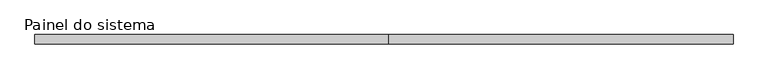
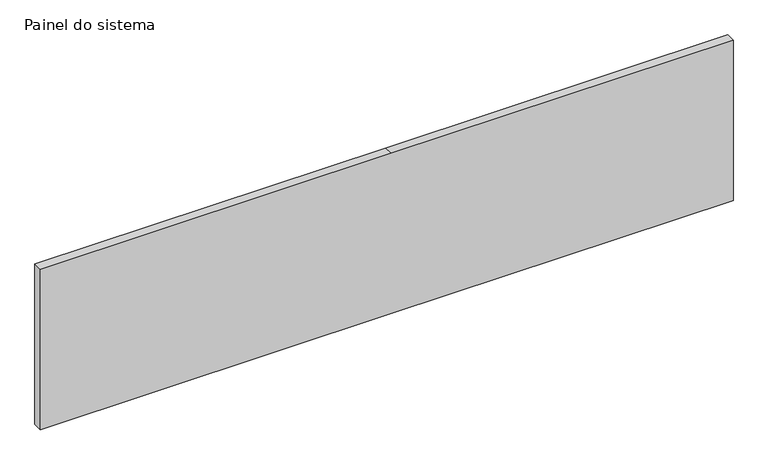
"""IFC4 building model written with IfcOpenShell, lengths in millimetres: plate geometry, Painel do sistema : Envidraçado."""

import ifcopenshell
import ifcopenshell.guid

model = None  # the IFC model being written
_history = None  # IfcOwnerHistory: only IFC2X3 demands one
_inside = {}  # id of a spatial element -> (the spatial element, [elements in it])
_under = {}  # id of a project, library or spatial element -> (it, [spatial elements below it])
_declared = {}  # id of a project -> (the project, [libraries it declares])
_typed = {}  # id of a type object -> (the type object, [elements of that type])
_made_of = {}  # id of a material, layer set ... -> (it, [elements and type objects made of it])


def new_model(schema):
    """Start an empty IFC model of exactly this schema.

    Asked for "IFC4X3", IfcOpenShell would pick the latest addendum, in which some entities
    have other attributes; the version numbers below select the first issue.
    IFC2X3 requires an IfcOwnerHistory on every rooted entity: one is made here for all.
    """
    global model, _history
    if schema == "IFC4X3":
        model = ifcopenshell.file(schema_version=(4, 3, 0, 0))
    else:
        model = ifcopenshell.file(schema=schema)
    _inside.clear()
    _under.clear()
    _declared.clear()
    _typed.clear()
    _made_of.clear()
    _history = None
    if model.schema == "IFC2X3":
        org = make("IfcOrganization", Name="unknown")
        user = make(
            "IfcPersonAndOrganization",
            ThePerson=make("IfcPerson", FamilyName="unknown"),
            TheOrganization=org,
        )
        app = make(
            "IfcApplication",
            ApplicationDeveloper=org,
            Version="unknown",
            ApplicationFullName="unknown",
            ApplicationIdentifier="unknown",
        )
        _history = make(
            "IfcOwnerHistory",
            OwningUser=user,
            OwningApplication=app,
            ChangeAction="ADDED",
            CreationDate=0,
        )
    return model


def make(cls, **values):
    """One entity of the class cls with the attributes given. An attribute that is None is left unset."""
    return model.create_entity(
        cls, **{name: value for name, value in values.items() if value is not None}
    )


def rooted(cls, **values):
    """An entity with a GlobalId (a new one), such as an element, a storey or a relation."""
    return make(cls, GlobalId=ifcopenshell.guid.new(), OwnerHistory=_history, **values)


def si_unit(unit_type, name, prefix=None):
    """IfcSIUnit, for example si_unit("LENGTHUNIT", "METRE", prefix="MILLI")."""
    return make("IfcSIUnit", UnitType=unit_type, Prefix=prefix, Name=name)


def assignment(units):
    """IfcUnitAssignment: the units of a project."""
    return None if units is None else make("IfcUnitAssignment", Units=units)


def point(xyz):
    """IfcCartesianPoint."""
    return None if xyz is None else make("IfcCartesianPoint", Coordinates=xyz)


def direction(xyz):
    """IfcDirection."""
    return None if xyz is None else make("IfcDirection", DirectionRatios=xyz)


def frame(location, z_axis=None, x_axis=None):
    """IfcAxis2Placement3D, a coordinate frame: its origin and axes. An axis left out is left unset."""
    return make(
        "IfcAxis2Placement3D",
        Location=point(location),
        Axis=direction(z_axis),
        RefDirection=direction(x_axis),
    )


def origin():
    """The frame at (0, 0, 0) with its axes left unset."""
    return frame((0.0, 0.0, 0.0))


def place(relative_to, where):
    """IfcLocalPlacement: puts the frame where relative to a parent placement (None: the world)."""
    return make(
        "IfcLocalPlacement", PlacementRelTo=relative_to, RelativePlacement=where
    )


def context(
    kind, dimensions, precision=None, world=None, true_north=None, identifier=None
):
    """IfcGeometricRepresentationContext, for example the 3D "Model" context."""
    return make(
        "IfcGeometricRepresentationContext",
        ContextIdentifier=identifier,
        ContextType=kind,
        CoordinateSpaceDimension=dimensions,
        Precision=precision,
        WorldCoordinateSystem=world,
        TrueNorth=true_north,
    )


def project(units=None, contexts=None):
    """IfcProject with its units and contexts."""
    return rooted(
        "IfcProject",
        Name="project",
        RepresentationContexts=contexts,
        UnitsInContext=assignment(units),
    )


def spatial(cls, under=None, at=None, **own):
    """A site, building, storey or space (cls), placed at a placement, below another one or the project."""
    s = rooted(cls, ObjectPlacement=at, **own)
    if under is not None:
        _under.setdefault(under.id(), (under, []))[1].append(s)
    return s


def polyline(points):
    """IfcPolyline through the points."""
    return make("IfcPolyline", Points=[point(p) for p in points])


def outline(outer, holes=None, kind="AREA"):
    """IfcArbitraryClosedProfileDef: a profile drawn as a closed curve; with holes, ...WithVoids."""
    if holes is None:
        return make("IfcArbitraryClosedProfileDef", ProfileType=kind, OuterCurve=outer)
    return make(
        "IfcArbitraryProfileDefWithVoids",
        ProfileType=kind,
        OuterCurve=outer,
        InnerCurves=holes,
    )


def extrude(swept, where, along, depth):
    """IfcExtrudedAreaSolid: the profile swept, set in the frame where, extruded along a direction by depth."""
    return make(
        "IfcExtrudedAreaSolid",
        SweptArea=swept,
        Position=where,
        ExtrudedDirection=direction(along),
        Depth=depth,
    )


def shape(context_of_items, identifier, shape_type, items):
    """IfcShapeRepresentation: the items that make up one representation, for example the "Body"."""
    return make(
        "IfcShapeRepresentation",
        ContextOfItems=context_of_items,
        RepresentationIdentifier=identifier,
        RepresentationType=shape_type,
        Items=items,
    )


def source(mapping_origin, context_of_items, identifier, shape_type, items):
    """IfcRepresentationMap: a shape defined once, which mapped items show again and again."""
    return make(
        "IfcRepresentationMap",
        MappingOrigin=mapping_origin,
        MappedRepresentation=shape(context_of_items, identifier, shape_type, items),
    )


def transform(
    local_origin,
    x_axis=None,
    y_axis=None,
    z_axis=None,
    scale=None,
    scale2=None,
    scale3=None,
    uniform=True,
):
    """IfcCartesianTransformationOperator3D, or its non-uniform kind. x_axis, y_axis, z_axis: its Axis1, 2, 3."""
    if uniform:
        return make(
            "IfcCartesianTransformationOperator3D",
            Axis1=direction(x_axis),
            Axis2=direction(y_axis),
            LocalOrigin=point(local_origin),
            Scale=scale,
            Axis3=direction(z_axis),
        )
    return make(
        "IfcCartesianTransformationOperator3DnonUniform",
        Axis1=direction(x_axis),
        Axis2=direction(y_axis),
        LocalOrigin=point(local_origin),
        Scale=scale,
        Axis3=direction(z_axis),
        Scale2=scale2,
        Scale3=scale3,
    )


def mapped(mapping_source, mapping_target):
    """IfcMappedItem: shows the shape of a source again, moved by a transform."""
    return make(
        "IfcMappedItem", MappingSource=mapping_source, MappingTarget=mapping_target
    )


def made_of(thing, what):
    """Note that an element or type object is made of a material, layer set ...; save() writes the relation."""
    if what is not None:
        _made_of.setdefault(what.id(), (what, []))[1].append(thing)
    return thing


def element(
    cls,
    number,
    at=None,
    inside=None,
    cuts=None,
    type_object=None,
    material=None,
    context=None,
    identifier="Body",
    shape_type=None,
    held_by="IfcProductDefinitionShape",
    body=None,
    shapes=None,
    **own,
):
    """One element of the class cls, such as IfcWall. Its Tag is "e" and its number.

    at: its placement. inside: the storey or other place that contains it. cuts: it is an
    opening in that element (IfcRelVoidsElement). A single representation is given by context,
    identifier, shape_type and body (its items); several are given by shapes. held_by: the class
    of the entity that holds the representations. save() writes the other relations.
    """
    e = rooted(cls, Tag="e%d" % number, ObjectPlacement=at, **own)
    if body is not None:
        shapes = [shape(context, identifier, shape_type, body)]
    if shapes is not None:
        e.Representation = make(held_by, Representations=shapes)
    if inside is not None:
        _inside.setdefault(inside.id(), (inside, []))[1].append(e)
    if cuts is not None:
        rooted(
            "IfcRelVoidsElement", RelatingBuildingElement=cuts, RelatedOpeningElement=e
        )
    if type_object is not None:
        _typed.setdefault(type_object.id(), (type_object, []))[1].append(e)
    return made_of(e, material)


def aggregate(whole, parts):
    """IfcRelAggregates: a whole, such as a stair, and the parts it consists of."""
    return rooted("IfcRelAggregates", RelatingObject=whole, RelatedObjects=parts)


def save(model, path):
    """Write the relations noted so far, then the file.

    IfcRelAggregates (storeys below a building ...), IfcRelContainedInSpatialStructure (elements
    in a storey), IfcRelDefinesByType, IfcRelAssociatesMaterial and IfcRelDeclares: one each for
    every whole, place, type object, material and project.
    """
    for whole, parts in _under.values():
        aggregate(whole, parts)
    for where, things in _inside.values():
        rooted(
            "IfcRelContainedInSpatialStructure",
            RelatedElements=things,
            RelatingStructure=where,
        )
    for kind, things in _typed.values():
        rooted("IfcRelDefinesByType", RelatedObjects=things, RelatingType=kind)
    for what, things in _made_of.values():
        rooted("IfcRelAssociatesMaterial", RelatedObjects=things, RelatingMaterial=what)
    for by, libraries in _declared.values():
        rooted("IfcRelDeclares", RelatingContext=by, RelatedDefinitions=libraries)
    model.write(path)


def painel_do_sistema_33a988d1(model_context):
    return source(origin(), model_context, "Body", "SweptSolid", [
        extrude(outline(polyline([(0.0, -918.5166667), (0.0, 12.4999998), (0.0, 918.5166667), (450.0, 918.5166667), (450.0, 12.4999998), (450.0, -918.5166667), (0.0, -918.5166667)])), frame((0.0, 24.5, 0.0), z_axis=(0.0, 1.0, 0.0), x_axis=(0.0, 0.0, 1.0)), (0.0, 0.0, 1.0), 25.0),
    ])


if __name__ == "__main__":
    model = new_model("IFC4")
    model_context = context("Model", 3, world=origin())
    ifc_project = project(units=[si_unit("LENGTHUNIT", "METRE", prefix="MILLI")], contexts=[model_context])
    site = spatial("IfcSite", under=ifc_project)
    building = spatial("IfcBuilding", under=site)
    placement = place(None, origin())
    painel_do_sistema_shape = painel_do_sistema_33a988d1(model_context)
    element("IfcPlate", 1, ObjectType="Painel do sistema : Envidraçado", at=placement, inside=building, context=model_context, shape_type="MappedRepresentation", body=[
        mapped(painel_do_sistema_shape, transform((0.0, 0.0, 0.0), x_axis=(1.0, 0.0, 0.0), y_axis=(0.0, 1.0, 0.0), z_axis=(0.0, 0.0, 1.0))),
    ])
    save(model, "model.ifc")

# Revit data of these elements
# Project information
#   Design Option = "Main Model"
#   Project Status = "Status do projeto"
#   Project Address = "RUA SÉRGIO DIAS, LOTE 30, QUADRA G, MONTE MINEIRO/MG"
#   Project Name = "RESIDÊNCIA - ROBERTA VENDRAMINI"
#   Project Number = "034/2017"
#   Zona = "ZER - 01"
#   CA Mín = "0.2"
#   CA Básico = "1"
#   CA Máx = "2"
#   TO Máx = "50"
#   Gabarito Máx = "10"
#   TP Mín = "15"
#   Área Total do Terreno = "620.00 m²"
#   Multifamiliar - Vagas Veículos/Pavto = "0"
#   Multifamiliar - Vagas Bicicletas/Pavto = "0"
#   Multifamiliar - % Vagas PNMR = "0"
#   Multifamiliar - % Vagas Motos = "0"
#   Outros - Área p/ 1 Veículo = "0.00 m²"
#   Outros - Área p/ 1 Bicicleta = "0.00 m²"
#   Outros - Área p/ 1 Utilitário = "0.00 m²"
#   Outros - % Vagas PNMR = "0"
#   Outros - % Vagas Motos = "0"
# Type "Painel do sistema : Envidraçado"
#   Construction Type Id = "GSP4R"
#   Analytic Construction = "Vidraça única Pilkington 1/8 pol"
#   Visual Light Transmittance = 0.9
#   Solar Heat Gain Coefficient = 0.86
#   Heat Transfer Coefficient (U) = 6.7069 W/(m²·K)
# Element 1 (IfcPlate, "Painel do sistema : Envidraçado")
#   Materials on its faces: ".VIDRO GENÉRICO"
# Materials
#   ".VIDRO GENÉRICO": class ".CC_VIDRO", colour RGB 0 128 192, transparency 0.9, Description = "Vidro comum", Cost = 0
